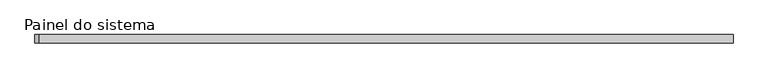
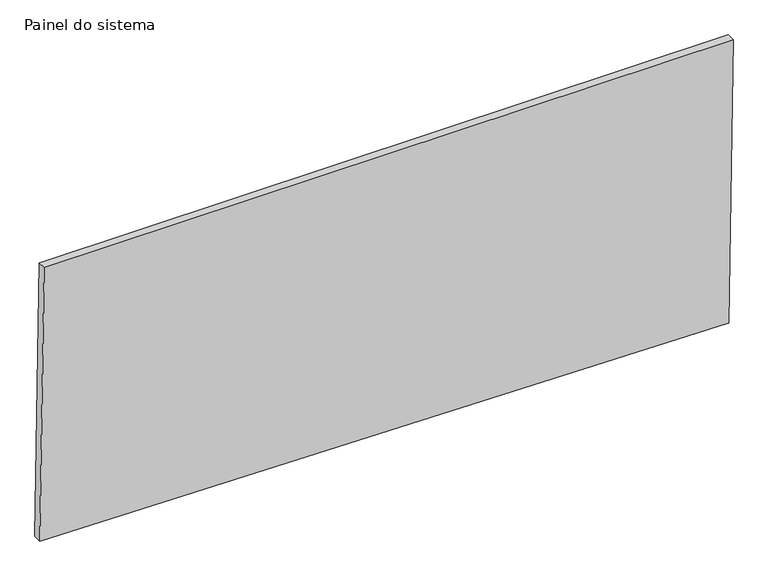
"""IFC4 building model written with IfcOpenShell, lengths in millimetres: plate geometry, Painel do sistema : Envidraçado."""

from ifc_helpers import new_model, si_unit, frame, origin, place, context, project, spatial, polyline, outline, extrude, source, transform, mapped, element, save


def painel_do_sistema_be4925aa(model_context):
    return source(origin(), model_context, "Body", "SweptSolid", [
        extrude(outline(polyline([(31.007472, -1037.5244966), (0.0, 1024.0976298), (892.7243631, 1037.5244966), (892.7243631, -1024.5639923), (31.007472, -1037.5244966)])), frame((0.0, 24.5, 0.0), z_axis=(0.0, 1.0, 0.0), x_axis=(0.0, 0.0, 1.0)), (0.0, 0.0, 1.0), 25.0),
    ])


if __name__ == "__main__":
    model = new_model("IFC4")
    model_context = context("Model", 3, world=origin())
    ifc_project = project(units=[si_unit("LENGTHUNIT", "METRE", prefix="MILLI")], contexts=[model_context])
    site = spatial("IfcSite", under=ifc_project)
    building = spatial("IfcBuilding", under=site)
    placement = place(None, origin())
    painel_do_sistema_shape = painel_do_sistema_be4925aa(model_context)
    element("IfcPlate", 1, ObjectType="Painel do sistema : Envidraçado", at=placement, inside=building, context=model_context, shape_type="MappedRepresentation", body=[
        mapped(painel_do_sistema_shape, transform((0.0, 0.0, 0.0), x_axis=(1.0, 0.0, 0.0), y_axis=(0.0, 1.0, 0.0), z_axis=(0.0, 0.0, 1.0))),
    ])
    save(model, "model.ifc")

# Revit data of these elements
# Type "Painel do sistema : Envidraçado"
#   Construction Type Id = "GSP4R"
#   Analytic Construction = "Vidraça única Pilkington 1/8 pol"
#   Visual Light Transmittance = 0.9
#   Solar Heat Gain Coefficient = 0.86
#   Heat Transfer Coefficient (U) = 6.7069 W/(m²·K)
# Element 1 (IfcPlate, "Painel do sistema : Envidraçado")
#   Materials on its faces: "Vidro"
# Materials
#   "Vidro": class "Vidro", colour RGB 0 128 192, transparency 0.9, Description = "Vidro de sílica", Cost = 0
